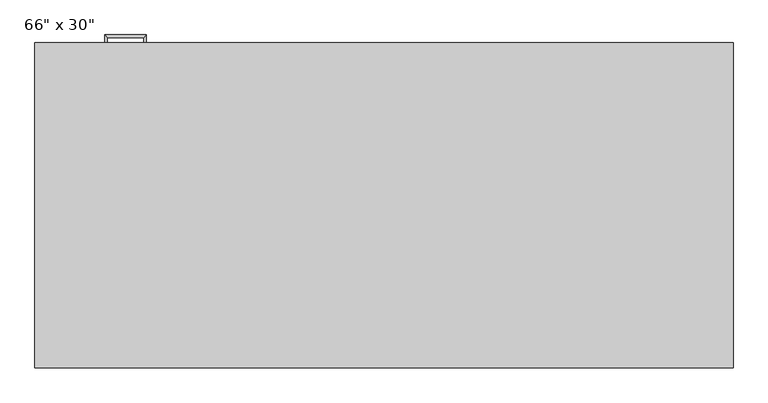
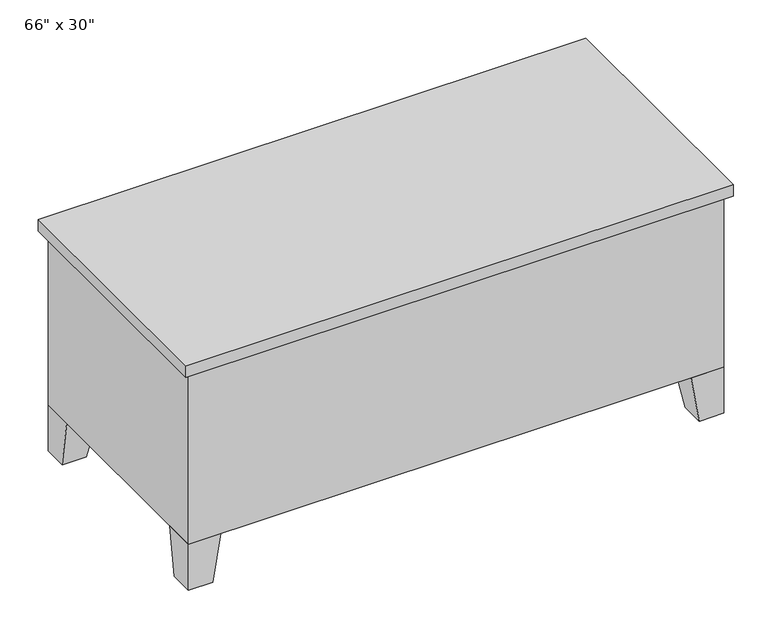
"""IFC4 building model written with IfcOpenShell, lengths in millimetres: furniture geometry."""

from ifc_helpers import new_model, si_unit, frame, origin, place, context, project, spatial, polyline, outline, extrude, faceted_brep, source, transform, mapped, element, save


def furniture_388a94df(model_context):
    return source(origin(), model_context, "Body", "SolidModel", [
        faceted_brep([(406.4, 762.0, 723.9), (0.0, 762.0, 723.9), (0.0, 0.0, 723.9), (1676.4, 0.0, 723.9), (1676.4, 762.0, 723.9), (1422.4, 762.0, 723.9), (1422.4, 50.8, 723.9), (406.4, 50.8, 723.9), (406.4, 762.0, 152.4), (406.4, 50.8, 152.4), (1422.4, 50.8, 152.4), (1422.4, 762.0, 152.4), (1676.4, 762.0, 152.4), (1676.4, 0.0, 152.4), (0.0, 0.0, 152.4), (0.0, 762.0, 152.4), (1441.45, 762.0, 171.45), (1657.35, 762.0, 171.45), (1657.35, 762.0, 704.85), (1441.45, 762.0, 704.85), (1441.45, 50.8, 171.45), (1441.45, 50.8, 704.85), (1657.35, 50.8, 704.85), (1657.35, 50.8, 171.45)], [[[0, 1, 2, 3, 4, 5, 6, 7]], [[8, 9, 10, 11, 12, 13, 14, 15]], [[1, 0, 8, 15]], [[2, 1, 15, 14]], [[3, 2, 14, 13]], [[4, 3, 13, 12]], [[5, 4, 12, 11], [16, 17, 18, 19]], [[6, 5, 11, 10]], [[7, 6, 10, 9]], [[0, 7, 9, 8]], [[20, 21, 22, 23]], [[20, 23, 17, 16]], [[23, 22, 18, 17]], [[22, 21, 19, 18]], [[21, 20, 16, 19]]]),
        extrude(outline(polyline([(387.35, 762.0), (19.05, 762.0), (19.05, 774.7), (387.35, 774.7), (387.35, 762.0)])), frame((0.0, 0.0, 603.25), z_axis=(0.0, 0.0, 1.0), x_axis=(1.0, 0.0, 0.0)), (0.0, 0.0, 1.0), 101.6),
        extrude(outline(polyline([(387.35, 762.0), (19.05, 762.0), (19.05, 774.7), (387.35, 774.7), (387.35, 762.0)])), frame((0.0, 0.0, 171.45), z_axis=(0.0, 0.0, 1.0), x_axis=(1.0, 0.0, 0.0)), (0.0, 0.0, 1.0), 171.45),
        extrude(outline(polyline([(387.35, 762.0), (19.05, 762.0), (19.05, 774.7), (387.35, 774.7), (387.35, 762.0)])), frame((0.0, 0.0, 482.6), z_axis=(0.0, 0.0, 1.0), x_axis=(1.0, 0.0, 0.0)), (0.0, 0.0, 1.0), 101.6),
        extrude(outline(polyline([(387.35, 762.0), (19.05, 762.0), (19.05, 774.7), (387.35, 774.7), (387.35, 762.0)])), frame((0.0, 0.0, 361.95), z_axis=(0.0, 0.0, 1.0), x_axis=(1.0, 0.0, 0.0)), (0.0, 0.0, 1.0), 101.6),
        faceted_brep([(1574.8, 762.0, 152.4), (1574.8, 660.4, 152.4), (1676.4, 660.4, 152.4), (1676.4, 762.0, 152.4), (1600.2, 762.0, 0.0), (1676.4, 762.0, 0.0), (1676.4, 685.8, 0.0), (1600.2, 685.8, 0.0)], [[[0, 1, 2, 3]], [[4, 5, 6, 7]], [[4, 7, 1, 0]], [[7, 6, 2, 1]], [[6, 5, 3, 2]], [[5, 4, 0, 3]]]),
        faceted_brep([(1574.8, 0.0, 152.4), (1676.4, 0.0, 152.4), (1676.4, 101.6, 152.4), (1574.8, 101.6, 152.4), (1600.2, 0.0, 0.0), (1600.2, 76.2, 0.0), (1676.4, 76.2, 0.0), (1676.4, 0.0, 0.0)], [[[0, 1, 2, 3]], [[4, 5, 6, 7]], [[4, 7, 1, 0]], [[7, 6, 2, 1]], [[6, 5, 3, 2]], [[5, 4, 0, 3]]]),
        faceted_brep([(101.6, 0.0, 152.4), (101.6, 101.6, 152.4), (0.0, 101.6, 152.4), (0.0, 0.0, 152.4), (76.2, 0.0, 0.0), (0.0, 0.0, 0.0), (0.0, 76.2, 0.0), (76.2, 76.2, 0.0)], [[[0, 1, 2, 3]], [[4, 5, 6, 7]], [[4, 7, 1, 0]], [[7, 6, 2, 1]], [[6, 5, 3, 2]], [[5, 4, 0, 3]]]),
        faceted_brep([(101.6, 762.0, 152.4), (0.0, 762.0, 152.4), (0.0, 660.4, 152.4), (101.6, 660.4, 152.4), (76.2, 762.0, 0.0), (76.2, 685.8, 0.0), (0.0, 685.8, 0.0), (0.0, 762.0, 0.0)], [[[0, 1, 2, 3]], [[4, 5, 6, 7]], [[4, 7, 1, 0]], [[7, 6, 2, 1]], [[6, 5, 3, 2]], [[5, 4, 0, 3]]]),
        extrude(outline(polyline([(1695.45, 781.05), (1695.45, -19.05), (-19.05, -19.05), (-19.05, 781.05), (1695.45, 781.05)])), frame((0.0, 0.0, 723.9), z_axis=(0.0, 0.0, 1.0), x_axis=(1.0, 0.0, 0.0)), (0.0, 0.0, 1.0), 38.1),
        faceted_brep([(158.75, 774.7, 304.8), (152.4, 774.7, 304.8), (152.4, 774.7, 292.1), (158.75, 774.7, 292.1), (158.75, 793.75, 304.8), (152.4, 800.1, 304.8), (152.4, 800.1, 292.1), (158.75, 793.75, 292.1), (247.65, 793.75, 304.8), (254.0, 800.1, 304.8), (254.0, 800.1, 292.1), (247.65, 793.75, 292.1), (247.65, 774.7, 304.8), (247.65, 774.7, 292.1), (254.0, 774.7, 292.1), (254.0, 774.7, 304.8)], [[[0, 1, 2, 3]], [[1, 0, 4, 5]], [[2, 1, 5, 6]], [[3, 2, 6, 7]], [[0, 3, 7, 4]], [[5, 4, 8, 9]], [[6, 5, 9, 10]], [[7, 6, 10, 11]], [[4, 7, 11, 8]], [[12, 13, 14, 15]], [[9, 8, 12, 15]], [[10, 9, 15, 14]], [[11, 10, 14, 13]], [[8, 11, 13, 12]]]),
        faceted_brep([(158.75, 774.7, 425.45), (152.4, 774.7, 425.45), (152.4, 774.7, 412.75), (158.75, 774.7, 412.75), (158.75, 793.75, 425.45), (152.4, 800.1, 425.45), (152.4, 800.1, 412.75), (158.75, 793.75, 412.75), (247.65, 793.75, 425.45), (254.0, 800.1, 425.45), (254.0, 800.1, 412.75), (247.65, 793.75, 412.75), (247.65, 774.7, 425.45), (247.65, 774.7, 412.75), (254.0, 774.7, 412.75), (254.0, 774.7, 425.45)], [[[0, 1, 2, 3]], [[1, 0, 4, 5]], [[2, 1, 5, 6]], [[3, 2, 6, 7]], [[0, 3, 7, 4]], [[5, 4, 8, 9]], [[6, 5, 9, 10]], [[7, 6, 10, 11]], [[4, 7, 11, 8]], [[12, 13, 14, 15]], [[9, 8, 12, 15]], [[10, 9, 15, 14]], [[11, 10, 14, 13]], [[8, 11, 13, 12]]]),
        faceted_brep([(158.75, 774.7, 546.1), (152.4, 774.7, 546.1), (152.4, 774.7, 533.4), (158.75, 774.7, 533.4), (158.75, 793.75, 546.1), (152.4, 800.1, 546.1), (152.4, 800.1, 533.4), (158.75, 793.75, 533.4), (247.65, 793.75, 546.1), (254.0, 800.1, 546.1), (254.0, 800.1, 533.4), (247.65, 793.75, 533.4), (247.65, 774.7, 546.1), (247.65, 774.7, 533.4), (254.0, 774.7, 533.4), (254.0, 774.7, 546.1)], [[[0, 1, 2, 3]], [[1, 0, 4, 5]], [[2, 1, 5, 6]], [[3, 2, 6, 7]], [[0, 3, 7, 4]], [[5, 4, 8, 9]], [[6, 5, 9, 10]], [[7, 6, 10, 11]], [[4, 7, 11, 8]], [[12, 13, 14, 15]], [[9, 8, 12, 15]], [[10, 9, 15, 14]], [[11, 10, 14, 13]], [[8, 11, 13, 12]]]),
        faceted_brep([(158.75, 774.7, 666.75), (152.4, 774.7, 666.75), (152.4, 774.7, 654.05), (158.75, 774.7, 654.05), (158.75, 793.75, 666.75), (152.4, 800.1, 666.75), (152.4, 800.1, 654.05), (158.75, 793.75, 654.05), (247.65, 793.75, 666.75), (254.0, 800.1, 666.75), (254.0, 800.1, 654.05), (247.65, 793.75, 654.05), (247.65, 774.7, 666.75), (247.65, 774.7, 654.05), (254.0, 774.7, 654.05), (254.0, 774.7, 666.75)], [[[0, 1, 2, 3]], [[1, 0, 4, 5]], [[2, 1, 5, 6]], [[3, 2, 6, 7]], [[0, 3, 7, 4]], [[5, 4, 8, 9]], [[6, 5, 9, 10]], [[7, 6, 10, 11]], [[4, 7, 11, 8]], [[12, 13, 14, 15]], [[9, 8, 12, 15]], [[10, 9, 15, 14]], [[11, 10, 14, 13]], [[8, 11, 13, 12]]]),
        extrude(outline(polyline([(1422.4, 381.0), (406.4, 381.0), (406.4, 762.0), (1422.4, 762.0), (1422.4, 381.0)])), frame((0.0, 0.0, 635.0), z_axis=(0.0, 0.0, 1.0), x_axis=(1.0, 0.0, 0.0)), (0.0, 0.0, 1.0), 19.05),
    ])


if __name__ == "__main__":
    model = new_model("IFC4")
    model_context = context("Model", 3, world=origin())
    ifc_project = project(units=[si_unit("LENGTHUNIT", "METRE", prefix="MILLI")], contexts=[model_context])
    site = spatial("IfcSite", under=ifc_project)
    building = spatial("IfcBuilding", under=site)
    placement = place(None, origin())
    furniture_shape = furniture_388a94df(model_context)
    element("IfcFurniture", 1, ObjectType="Desk-Secretary : 66\" x 30\"", at=placement, inside=building, context=model_context, shape_type="MappedRepresentation", body=[
        mapped(furniture_shape, transform((0.0, 0.0, 0.0), x_axis=(1.0, 0.0, 0.0), y_axis=(0.0, 1.0, 0.0), z_axis=(0.0, 0.0, 1.0))),
    ])
    save(model, "model.ifc")

# Revit data of these elements
# Type "Desk-Secretary : 66\" x 30\""
#   Model = "SEC-4567"
#   Manufacturer = "Furniture Concepts"
#   Type Mark = "DK-3"
#   Model = "SEC-4567"
#   Manufacturer = "Furniture Concepts"
#   Assembly Code = "E2020200"
#   Cost = 895
#   Cost = 895
#   Depth = 2' - 6"
#   Height = 2' - 6"
#   Leg Height = 0' - 6"
#   Width = 5' - 6"
#   Type Image = Secretarial Desk.png
#   Body Material = Laminate, Ivory, Matte
#   Handle/Leg Material = Steel, Chrome Plated
#   Top Material = Cherry
#   Default Elevation = 0
# Element 1 (IfcFurniture, "Desk-Secretary : 66\" x 30\"")
#   Materials on its faces: "Steel, Chrome Plated", "Laminate, Ivory, Matte", "Cherry"
# Materials
#   "Laminate, Ivory, Matte": class "Plastic", colour RGB 247 247 239, transparency 0, Description = "Plastic Laminate - Ivory, Matte", Cost = 0
#   "Steel, Chrome Plated": class "Metal", colour RGB 17 17 17, transparency 0, Description = "Chromiuim plated steel", Cost = 0
#   "Cherry": class "Wood", colour RGB 226 177 128, transparency 0, Description = "Prunus Serotina", Cost = 0
